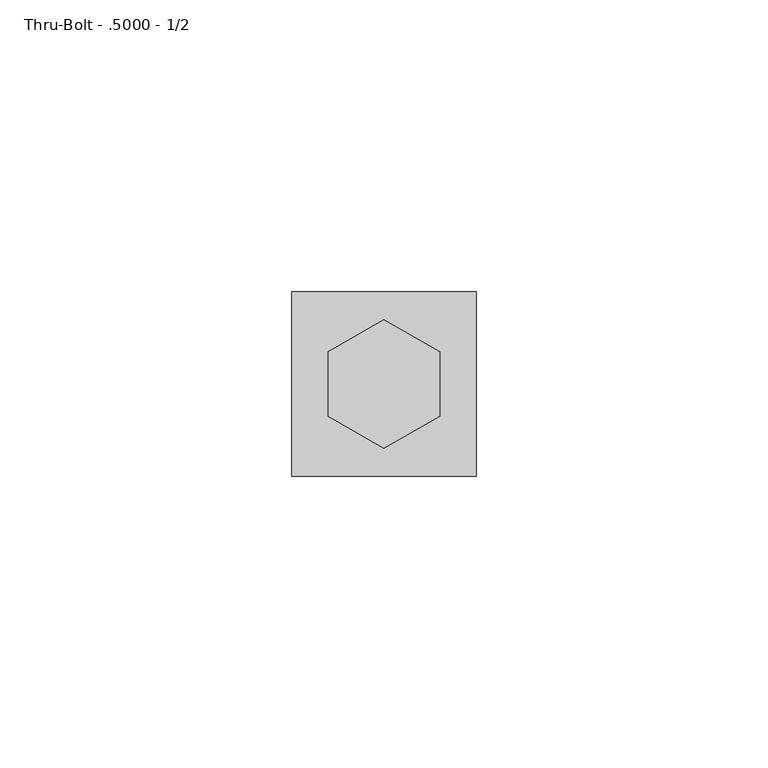
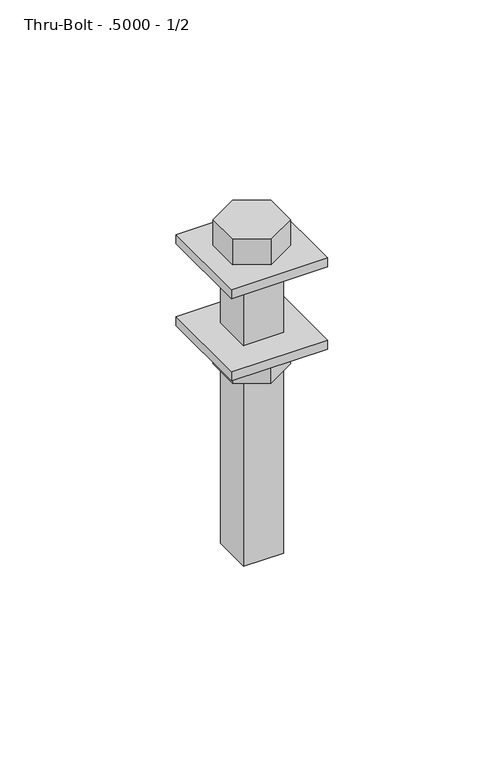
"""IFC4 building model written with IfcOpenShell, lengths in millimetres: fastener geometry, 060523 - W_P_C - Fastenings - Generic - SQUARE : Thru-Bolt - .5000 - 1/2."""

import ifcopenshell
import ifcopenshell.guid

model = None  # the IFC model being written
_history = None  # IfcOwnerHistory: only IFC2X3 demands one
_inside = {}  # id of a spatial element -> (the spatial element, [elements in it])
_under = {}  # id of a project, library or spatial element -> (it, [spatial elements below it])
_declared = {}  # id of a project -> (the project, [libraries it declares])
_typed = {}  # id of a type object -> (the type object, [elements of that type])
_made_of = {}  # id of a material, layer set ... -> (it, [elements and type objects made of it])


def new_model(schema):
    """Start an empty IFC model of exactly this schema.

    Asked for "IFC4X3", IfcOpenShell would pick the latest addendum, in which some entities
    have other attributes; the version numbers below select the first issue.
    IFC2X3 requires an IfcOwnerHistory on every rooted entity: one is made here for all.
    """
    global model, _history
    if schema == "IFC4X3":
        model = ifcopenshell.file(schema_version=(4, 3, 0, 0))
    else:
        model = ifcopenshell.file(schema=schema)
    _inside.clear()
    _under.clear()
    _declared.clear()
    _typed.clear()
    _made_of.clear()
    _history = None
    if model.schema == "IFC2X3":
        org = make("IfcOrganization", Name="unknown")
        user = make(
            "IfcPersonAndOrganization",
            ThePerson=make("IfcPerson", FamilyName="unknown"),
            TheOrganization=org,
        )
        app = make(
            "IfcApplication",
            ApplicationDeveloper=org,
            Version="unknown",
            ApplicationFullName="unknown",
            ApplicationIdentifier="unknown",
        )
        _history = make(
            "IfcOwnerHistory",
            OwningUser=user,
            OwningApplication=app,
            ChangeAction="ADDED",
            CreationDate=0,
        )
    return model


def make(cls, **values):
    """One entity of the class cls with the attributes given. An attribute that is None is left unset."""
    return model.create_entity(
        cls, **{name: value for name, value in values.items() if value is not None}
    )


def rooted(cls, **values):
    """An entity with a GlobalId (a new one), such as an element, a storey or a relation."""
    return make(cls, GlobalId=ifcopenshell.guid.new(), OwnerHistory=_history, **values)


def si_unit(unit_type, name, prefix=None):
    """IfcSIUnit, for example si_unit("LENGTHUNIT", "METRE", prefix="MILLI")."""
    return make("IfcSIUnit", UnitType=unit_type, Prefix=prefix, Name=name)


def assignment(units):
    """IfcUnitAssignment: the units of a project."""
    return None if units is None else make("IfcUnitAssignment", Units=units)


def point(xyz):
    """IfcCartesianPoint."""
    return None if xyz is None else make("IfcCartesianPoint", Coordinates=xyz)


def direction(xyz):
    """IfcDirection."""
    return None if xyz is None else make("IfcDirection", DirectionRatios=xyz)


def frame(location, z_axis=None, x_axis=None):
    """IfcAxis2Placement3D, a coordinate frame: its origin and axes. An axis left out is left unset."""
    return make(
        "IfcAxis2Placement3D",
        Location=point(location),
        Axis=direction(z_axis),
        RefDirection=direction(x_axis),
    )


def origin():
    """The frame at (0, 0, 0) with its axes left unset."""
    return frame((0.0, 0.0, 0.0))


def origin_with_axes():
    """The frame at (0, 0, 0) with the z axis (0, 0, 1) and the x axis (1, 0, 0) written out."""
    return frame((0.0, 0.0, 0.0), z_axis=(0.0, 0.0, 1.0), x_axis=(1.0, 0.0, 0.0))


def place(relative_to, where):
    """IfcLocalPlacement: puts the frame where relative to a parent placement (None: the world)."""
    return make(
        "IfcLocalPlacement", PlacementRelTo=relative_to, RelativePlacement=where
    )


def context(
    kind, dimensions, precision=None, world=None, true_north=None, identifier=None
):
    """IfcGeometricRepresentationContext, for example the 3D "Model" context."""
    return make(
        "IfcGeometricRepresentationContext",
        ContextIdentifier=identifier,
        ContextType=kind,
        CoordinateSpaceDimension=dimensions,
        Precision=precision,
        WorldCoordinateSystem=world,
        TrueNorth=true_north,
    )


def project(units=None, contexts=None):
    """IfcProject with its units and contexts."""
    return rooted(
        "IfcProject",
        Name="project",
        RepresentationContexts=contexts,
        UnitsInContext=assignment(units),
    )


def spatial(cls, under=None, at=None, **own):
    """A site, building, storey or space (cls), placed at a placement, below another one or the project."""
    s = rooted(cls, ObjectPlacement=at, **own)
    if under is not None:
        _under.setdefault(under.id(), (under, []))[1].append(s)
    return s


def polyline(points):
    """IfcPolyline through the points."""
    return make("IfcPolyline", Points=[point(p) for p in points])


def outline(outer, holes=None, kind="AREA"):
    """IfcArbitraryClosedProfileDef: a profile drawn as a closed curve; with holes, ...WithVoids."""
    if holes is None:
        return make("IfcArbitraryClosedProfileDef", ProfileType=kind, OuterCurve=outer)
    return make(
        "IfcArbitraryProfileDefWithVoids",
        ProfileType=kind,
        OuterCurve=outer,
        InnerCurves=holes,
    )


def extrude(swept, where, along, depth):
    """IfcExtrudedAreaSolid: the profile swept, set in the frame where, extruded along a direction by depth."""
    return make(
        "IfcExtrudedAreaSolid",
        SweptArea=swept,
        Position=where,
        ExtrudedDirection=direction(along),
        Depth=depth,
    )


def shape(context_of_items, identifier, shape_type, items):
    """IfcShapeRepresentation: the items that make up one representation, for example the "Body"."""
    return make(
        "IfcShapeRepresentation",
        ContextOfItems=context_of_items,
        RepresentationIdentifier=identifier,
        RepresentationType=shape_type,
        Items=items,
    )


def source(mapping_origin, context_of_items, identifier, shape_type, items):
    """IfcRepresentationMap: a shape defined once, which mapped items show again and again."""
    return make(
        "IfcRepresentationMap",
        MappingOrigin=mapping_origin,
        MappedRepresentation=shape(context_of_items, identifier, shape_type, items),
    )


def transform(
    local_origin,
    x_axis=None,
    y_axis=None,
    z_axis=None,
    scale=None,
    scale2=None,
    scale3=None,
    uniform=True,
):
    """IfcCartesianTransformationOperator3D, or its non-uniform kind. x_axis, y_axis, z_axis: its Axis1, 2, 3."""
    if uniform:
        return make(
            "IfcCartesianTransformationOperator3D",
            Axis1=direction(x_axis),
            Axis2=direction(y_axis),
            LocalOrigin=point(local_origin),
            Scale=scale,
            Axis3=direction(z_axis),
        )
    return make(
        "IfcCartesianTransformationOperator3DnonUniform",
        Axis1=direction(x_axis),
        Axis2=direction(y_axis),
        LocalOrigin=point(local_origin),
        Scale=scale,
        Axis3=direction(z_axis),
        Scale2=scale2,
        Scale3=scale3,
    )


def mapped(mapping_source, mapping_target):
    """IfcMappedItem: shows the shape of a source again, moved by a transform."""
    return make(
        "IfcMappedItem", MappingSource=mapping_source, MappingTarget=mapping_target
    )


def made_of(thing, what):
    """Note that an element or type object is made of a material, layer set ...; save() writes the relation."""
    if what is not None:
        _made_of.setdefault(what.id(), (what, []))[1].append(thing)
    return thing


def element(
    cls,
    number,
    at=None,
    inside=None,
    cuts=None,
    type_object=None,
    material=None,
    context=None,
    identifier="Body",
    shape_type=None,
    held_by="IfcProductDefinitionShape",
    body=None,
    shapes=None,
    **own,
):
    """One element of the class cls, such as IfcWall. Its Tag is "e" and its number.

    at: its placement. inside: the storey or other place that contains it. cuts: it is an
    opening in that element (IfcRelVoidsElement). A single representation is given by context,
    identifier, shape_type and body (its items); several are given by shapes. held_by: the class
    of the entity that holds the representations. save() writes the other relations.
    """
    e = rooted(cls, Tag="e%d" % number, ObjectPlacement=at, **own)
    if body is not None:
        shapes = [shape(context, identifier, shape_type, body)]
    if shapes is not None:
        e.Representation = make(held_by, Representations=shapes)
    if inside is not None:
        _inside.setdefault(inside.id(), (inside, []))[1].append(e)
    if cuts is not None:
        rooted(
            "IfcRelVoidsElement", RelatingBuildingElement=cuts, RelatedOpeningElement=e
        )
    if type_object is not None:
        _typed.setdefault(type_object.id(), (type_object, []))[1].append(e)
    return made_of(e, material)


def aggregate(whole, parts):
    """IfcRelAggregates: a whole, such as a stair, and the parts it consists of."""
    return rooted("IfcRelAggregates", RelatingObject=whole, RelatedObjects=parts)


def save(model, path):
    """Write the relations noted so far, then the file.

    IfcRelAggregates (storeys below a building ...), IfcRelContainedInSpatialStructure (elements
    in a storey), IfcRelDefinesByType, IfcRelAssociatesMaterial and IfcRelDeclares: one each for
    every whole, place, type object, material and project.
    """
    for whole, parts in _under.values():
        aggregate(whole, parts)
    for where, things in _inside.values():
        rooted(
            "IfcRelContainedInSpatialStructure",
            RelatedElements=things,
            RelatingStructure=where,
        )
    for kind, things in _typed.values():
        rooted("IfcRelDefinesByType", RelatedObjects=things, RelatingType=kind)
    for what, things in _made_of.values():
        rooted("IfcRelAssociatesMaterial", RelatedObjects=things, RelatingMaterial=what)
    for by, libraries in _declared.values():
        rooted("IfcRelDeclares", RelatingContext=by, RelatedDefinitions=libraries)
    model.write(path)


def thru_bolt_5000_1_2_b29ce19b(model_context):
    return source(origin(), model_context, "Body", "SweptSolid", [
        extrude(outline(polyline([(-15.7757813, -15.7757813), (-15.7757813, 15.7757812), (15.7757812, 15.7757812), (15.7757812, -15.7757813), (-15.7757813, -15.7757813)])), origin_with_axes(), (0.0, 0.0, 1.0), 3.0757812),
        extrude(outline(polyline([(-15.7757813, -15.7757813), (-15.7757813, 15.7757812), (15.7757812, 15.7757812), (15.7757812, -15.7757813), (-15.7757813, -15.7757813)])), frame((0.0, 0.0, -28.4757813), z_axis=(0.0, 0.0, 1.0), x_axis=(1.0, 0.0, 0.0)), (0.0, 0.0, 1.0), 3.0757812),
        extrude(outline(polyline([(-9.525, -5.4992613), (-9.525, 5.4992613), (0.0, 10.9985226), (9.525, 5.4992613), (9.525, -5.4992613), (0.0, -10.9985226), (-9.525, -5.4992613)])), frame((0.0, 0.0, -37.703125), z_axis=(0.0, 0.0, 1.0), x_axis=(1.0, 0.0, 0.0)), (0.0, 0.0, 1.0), 9.2273437),
        extrude(outline(polyline([(-9.525, 5.4992613), (0.0, 10.9985226), (9.525, 5.4992613), (9.525, -5.4992613), (0.0, -10.9985226), (-9.525, -5.4992613), (-9.525, 5.4992613)])), frame((0.0, 0.0, 3.0757813), z_axis=(0.0, 0.0, 1.0), x_axis=(1.0, 0.0, 0.0)), (0.0, 0.0, 1.0), 9.2273437),
        extrude(outline(polyline([(-6.5484375, 6.5484375), (6.5484375, 6.5484375), (6.5484375, -6.5484375), (-6.5484375, -6.5484375), (-6.5484375, 6.5484375)])), frame((0.0, 0.0, -101.6), z_axis=(0.0, 0.0, 1.0), x_axis=(1.0, 0.0, 0.0)), (0.0, 0.0, 1.0), 104.6757812),
    ])


if __name__ == "__main__":
    model = new_model("IFC4")
    model_context = context("Model", 3, world=origin())
    ifc_project = project(units=[si_unit("LENGTHUNIT", "METRE", prefix="MILLI")], contexts=[model_context])
    site = spatial("IfcSite", under=ifc_project)
    building = spatial("IfcBuilding", under=site)
    placement = place(None, origin())
    thru_bolt_5000_1_2_shape = thru_bolt_5000_1_2_b29ce19b(model_context)
    element("IfcFastener", 1, ObjectType="060523 - W_P_C - Fastenings - Generic - SQUARE : Thru-Bolt - .5000 - 1/2", at=placement, inside=building, context=model_context, shape_type="MappedRepresentation", body=[
        mapped(thru_bolt_5000_1_2_shape, transform((0.0, 0.0, 0.0), x_axis=(1.0, 0.0, 0.0), y_axis=(0.0, 1.0, 0.0), z_axis=(0.0, 0.0, 1.0))),
    ])
    save(model, "model.ifc")

# Revit data of these elements
# Type "060523 - W_P_C - Fastenings - Generic - SQUARE : Thru-Bolt - .5000 - 1/2"
#   Washer_Thickness = 0' - 0 31/256"
#   Washer Radius = 0' - 0 159/256"
#   Washer Offset - Head = 0' - 0 31/256"
#   Washer Offset = 0' - 0 31/256"
#   Thickness_of_Substrate [instance default] = 0' - 1"
#   Side = 0' - 0 111/256"
#   Radius = 0' - 0 33/128"
#   Length [instance default] = 0' - 4"
#   Head Size = 0' - 0 3/4"
#   Head Radius = 0' - 0 3/8"
#   Head Height = 0' - 0 93/256"
#   Double Diameter = 0' - 1 1/32"
#   Diameter = 0' - 0 33/64"
#   Default Elevation = 4' - 0"
#   Washer_Nut_Visibility = yes
#   Washer_Head_Visibility = yes
#   Round_Head_Visibility = no
#   Point Visibility = no
#   Nut_Visibility = yes
#   Hex_Head_Visiblilty = yes
#   Washer Material = none
#   Bolt Material (Size) = AT SILL - FASTENER AT 24" O.C.
# Element 1 (IfcFastener, "060523 - W_P_C - Fastenings - Generic - SQUARE : Thru-Bolt - .5000 - 1/2")
#   Materials on its faces: "AT SILL - FASTENER AT 24\" O.C."
# Materials
#   "AT SILL - FASTENER AT 24\" O.C.": class "Generic", colour RGB 120 120 120, transparency 0, Cost = 0
